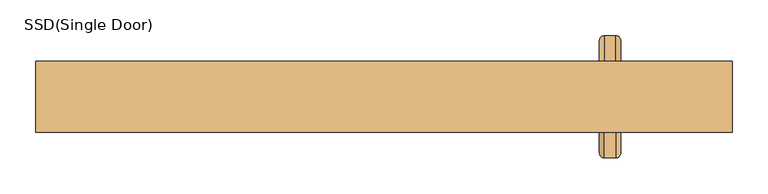
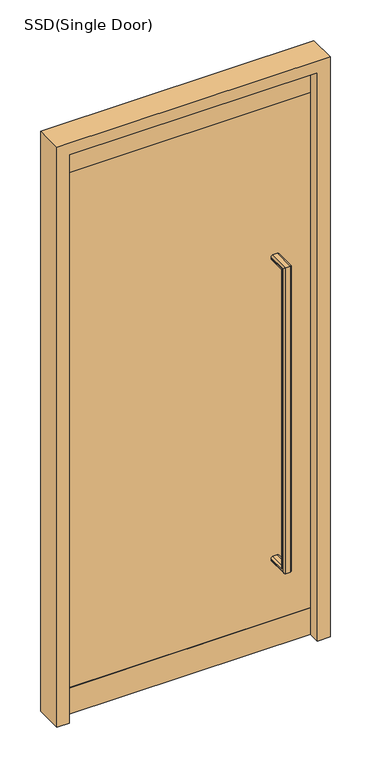
"""IFC4 building model written with IfcOpenShell, lengths in millimetres: door geometry, SSD(Single Door) : H_DR_AR B12_Door_Single_Glass_W1000xH2200_SSD-1."""

from ifc_helpers import new_model, si_unit, frame, origin, origin_with_axes, place, context, project, spatial, polyline, circle_curve, ellipse_curve, outline, extrude, source, transform, mapped, element, save
from ifc_brep_helpers import plane_surface, cylinder_surface, advanced_brep


def ssd_single_door_4e4cf73e(model_context):
    return source(origin(), model_context, "Body", "SolidModel", [
        extrude(outline(polyline([(0.0, -490.0), (0.0, -445.0), (2155.0, -445.0), (2155.0, 445.0), (0.0, 445.0), (0.0, 490.0), (2200.0, 490.0), (2200.0, -490.0), (0.0, -490.0)])), frame((0.0, -50.0, 0.0), z_axis=(0.0, 1.0, 0.0), x_axis=(0.0, 0.0, 1.0)), (0.0, 0.0, 1.0), 100.0),
        advanced_brep(
        [(310.0, -6.0, 1485.0), (326.0, -6.0, 1485.0), (333.0, -6.0, 1478.0), (333.0, -6.0, 1475.0), (326.0, -6.0, 1468.0), (310.0, -6.0, 1468.0), (303.0, -6.0, 1475.0), (303.0, -6.0, 1478.0), (310.0, -6.0, 325.0), (303.0, -6.0, 332.0), (303.0, -6.0, 335.0), (310.0, -6.0, 342.0), (326.0, -6.0, 342.0), (333.0, -6.0, 335.0), (333.0, -6.0, 332.0), (326.0, -6.0, 325.0), (310.0, -86.0, 1485.0), (326.0, -86.0, 1485.0), (333.0, -79.0, 1478.0), (333.0, -79.0, 332.0), (333.0, -76.0, 335.0), (333.0, -76.0, 1475.0), (326.0, -69.0, 1468.0), (310.0, -69.0, 1468.0), (303.0, -76.0, 1475.0), (303.0, -76.0, 335.0), (303.0, -79.0, 332.0), (303.0, -79.0, 1478.0), (310.0, -86.0, 325.0), (326.0, -86.0, 325.0), (326.0, -69.0, 342.0), (310.0, -69.0, 342.0)],
        [
            (0, 1),
            (1, 2, circle_curve(frame((326.0, -6.0, 1478.0), z_axis=(0.0, 1.0, 0.0), x_axis=(0.0, 0.0, -1.0)), 7.0)),
            (2, 3),
            (3, 4, circle_curve(frame((326.0, -6.0, 1475.0), z_axis=(0.0, 1.0, 0.0), x_axis=(0.0, 0.0, -1.0)), 7.0)),
            (4, 5),
            (5, 6, circle_curve(frame((310.0, -6.0, 1475.0), z_axis=(0.0, 1.0, 0.0), x_axis=(0.0, 0.0, -1.0)), 7.0)),
            (6, 7),
            (7, 0, circle_curve(frame((310.0, -6.0, 1478.0), z_axis=(0.0, 1.0, 0.0), x_axis=(0.0, 0.0, -1.0)), 7.0)),
            (8, 9, circle_curve(frame((310.0, -6.0, 332.0), z_axis=(0.0, 1.0, 0.0), x_axis=(0.0, 0.0, 1.0)), 7.0)),
            (9, 10),
            (10, 11, circle_curve(frame((310.0, -6.0, 335.0), z_axis=(0.0, 1.0, 0.0), x_axis=(0.0, 0.0, 1.0)), 7.0)),
            (11, 12),
            (12, 13, circle_curve(frame((326.0, -6.0, 335.0), z_axis=(0.0, 1.0, 0.0), x_axis=(0.0, 0.0, 1.0)), 7.0)),
            (13, 14),
            (14, 15, circle_curve(frame((326.0, -6.0, 332.0), z_axis=(0.0, 1.0, 0.0), x_axis=(0.0, 0.0, 1.0)), 7.0)),
            (15, 8),
            (0, 16),
            (16, 17),
            (17, 1),
            (17, 18, ellipse_curve(frame((326.0, -79.0, 1478.0), z_axis=(0.0, 0.7071067811865475, 0.7071067811865475), x_axis=(0.0, 0.7071067811865476, -0.7071067811865474)), 9.8994949, 7.0)),
            (18, 2),
            (18, 19),
            (19, 14),
            (13, 20),
            (20, 21),
            (21, 3),
            (21, 22, ellipse_curve(frame((326.0, -76.0, 1475.0), z_axis=(0.0, 0.7071067811865475, 0.7071067811865475), x_axis=(0.0, 0.7071067811865476, -0.7071067811865474)), 9.8994949, 7.0)),
            (22, 4),
            (22, 23),
            (23, 5),
            (23, 24, ellipse_curve(frame((310.0, -76.0, 1475.0), z_axis=(0.0, 0.7071067811865475, 0.7071067811865475), x_axis=(0.0, 0.7071067811865476, -0.7071067811865474)), 9.8994949, 7.0)),
            (24, 6),
            (24, 25),
            (25, 10),
            (9, 26),
            (26, 27),
            (27, 7),
            (27, 16, ellipse_curve(frame((310.0, -79.0, 1478.0), z_axis=(0.0, 0.7071067811865475, 0.7071067811865475), x_axis=(0.0, 0.7071067811865476, -0.7071067811865474)), 9.8994949, 7.0)),
            (16, 28),
            (28, 29),
            (29, 17),
            (29, 19, ellipse_curve(frame((326.0, -79.0, 332.0), z_axis=(0.0, -0.7071067811865475, 0.7071067811865475), x_axis=(0.0, 0.7071067811865474, 0.7071067811865476)), 9.8994949, 7.0)),
            (20, 30, ellipse_curve(frame((326.0, -76.0, 335.0), z_axis=(0.0, -0.7071067811865475, 0.7071067811865475), x_axis=(0.0, 0.7071067811865474, 0.7071067811865476)), 9.8994949, 7.0)),
            (30, 22),
            (30, 31),
            (31, 23),
            (31, 25, ellipse_curve(frame((310.0, -76.0, 335.0), z_axis=(0.0, -0.7071067811865475, 0.7071067811865475), x_axis=(0.0, 0.7071067811865474, 0.7071067811865476)), 9.8994949, 7.0)),
            (26, 28, ellipse_curve(frame((310.0, -79.0, 332.0), z_axis=(0.0, -0.7071067811865475, 0.7071067811865475), x_axis=(0.0, 0.7071067811865474, 0.7071067811865476)), 9.8994949, 7.0)),
            (28, 8),
            (15, 29),
            (12, 30),
            (11, 31),
        ],
        [
            plane_surface(frame((0.0, -6.0, 1485.0), z_axis=(0.0, 1.0, 0.0), x_axis=(1.0, 0.0, 0.0))),
            plane_surface(frame((0.0, -6.0, 325.0), z_axis=(0.0, 1.0, 0.0), x_axis=(1.0, 0.0, 0.0))),
            plane_surface(frame((310.0, -6.0, 1485.0), z_axis=(0.0, 0.0, 1.0), x_axis=(0.0, -1.0, 0.0))),
            cylinder_surface(frame((326.0, -6.0, 1478.0), z_axis=(0.0, 1.0, 0.0), x_axis=(0.0, 0.0, -1.0)), 7.0),
            plane_surface(frame((333.0, -6.0, 1478.0), z_axis=(1.0, 0.0, 0.0), x_axis=(0.0, -1.0, 0.0))),
            cylinder_surface(frame((326.0, -6.0, 1475.0), z_axis=(0.0, 1.0, 0.0), x_axis=(0.0, 0.0, -1.0)), 7.0),
            plane_surface(frame((326.0, -6.0, 1468.0), z_axis=(0.0, 0.0, -1.0), x_axis=(0.0, -1.0, 0.0))),
            cylinder_surface(frame((310.0, -6.0, 1475.0), z_axis=(0.0, 1.0, 0.0), x_axis=(0.0, 0.0, -1.0)), 7.0),
            plane_surface(frame((303.0, -6.0, 1475.0), z_axis=(-1.0, 0.0, 0.0), x_axis=(0.0, -1.0, 0.0))),
            cylinder_surface(frame((310.0, -6.0, 1478.0), z_axis=(0.0, 1.0, 0.0), x_axis=(0.0, 0.0, -1.0)), 7.0),
            plane_surface(frame((310.0, -86.0, 1485.0), z_axis=(0.0, -1.0, 0.0), x_axis=(0.0, 0.0, -1.0))),
            cylinder_surface(frame((326.0, -79.0, 1485.0), z_axis=(0.0, 0.0, 1.0), x_axis=(0.0, 1.0, 0.0)), 7.0),
            cylinder_surface(frame((326.0, -76.0, 1485.0), z_axis=(0.0, 0.0, 1.0), x_axis=(0.0, 1.0, 0.0)), 7.0),
            plane_surface(frame((326.0, -69.0, 1468.0), z_axis=(0.0, 1.0, 0.0), x_axis=(0.0, 0.0, -1.0))),
            cylinder_surface(frame((310.0, -76.0, 1485.0), z_axis=(0.0, 0.0, 1.0), x_axis=(0.0, 1.0, 0.0)), 7.0),
            cylinder_surface(frame((310.0, -79.0, 1485.0), z_axis=(0.0, 0.0, 1.0), x_axis=(0.0, 1.0, 0.0)), 7.0),
            plane_surface(frame((310.0, -86.0, 325.0), z_axis=(0.0, 0.0, -1.0), x_axis=(0.0, 1.0, 0.0))),
            cylinder_surface(frame((326.0, -86.0, 332.0), z_axis=(0.0, -1.0, 0.0), x_axis=(0.0, 0.0, 1.0)), 7.0),
            cylinder_surface(frame((326.0, -86.0, 335.0), z_axis=(0.0, -1.0, 0.0), x_axis=(0.0, 0.0, 1.0)), 7.0),
            plane_surface(frame((326.0, -69.0, 342.0), z_axis=(0.0, 0.0, 1.0), x_axis=(0.0, 1.0, 0.0))),
            cylinder_surface(frame((310.0, -86.0, 335.0), z_axis=(0.0, -1.0, 0.0), x_axis=(0.0, 0.0, 1.0)), 7.0),
            cylinder_surface(frame((310.0, -86.0, 332.0), z_axis=(0.0, -1.0, 0.0), x_axis=(0.0, 0.0, 1.0)), 7.0),
        ],
        [
            (0, [[1, 2, 3, 4, 5, 6, 7, 8]]),
            (1, [[9, 10, 11, 12, 13, 14, 15, 16]]),
            (2, [[-1, 17, 18, 19]]),
            (3, [[-2, -19, 20, 21]]),
            (4, [[-3, -21, 22, 23, -14, 24, 25, 26]]),
            (5, [[-4, -26, 27, 28]]),
            (6, [[-5, -28, 29, 30]]),
            (7, [[-6, -30, 31, 32]]),
            (8, [[-7, -32, 33, 34, -10, 35, 36, 37]]),
            (9, [[-8, -37, 38, -17]]),
            (10, [[-18, 39, 40, 41]]),
            (11, [[-20, -41, 42, -22]]),
            (12, [[-27, -25, 43, 44]]),
            (13, [[-29, -44, 45, 46]]),
            (14, [[-31, -46, 47, -33]]),
            (15, [[-38, -36, 48, -39]]),
            (16, [[-40, 49, -16, 50]]),
            (17, [[-42, -50, -15, -23]]),
            (18, [[-43, -24, -13, 51]]),
            (19, [[-45, -51, -12, 52]]),
            (20, [[-47, -52, -11, -34]]),
            (21, [[-48, -35, -9, -49]]),
        ],
    ),
        advanced_brep(
        [(310.0, 6.0, 1485.0), (303.0, 6.0, 1478.0), (303.0, 6.0, 1475.0), (310.0, 6.0, 1468.0), (326.0, 6.0, 1468.0), (333.0, 6.0, 1475.0), (333.0, 6.0, 1478.0), (326.0, 6.0, 1485.0), (310.0, 6.0, 325.0), (326.0, 6.0, 325.0), (333.0, 6.0, 332.0), (333.0, 6.0, 335.0), (326.0, 6.0, 342.0), (310.0, 6.0, 342.0), (303.0, 6.0, 335.0), (303.0, 6.0, 332.0), (310.0, 86.0, 1485.0), (303.0, 79.0, 1478.0), (303.0, 79.0, 332.0), (303.0, 76.0, 335.0), (303.0, 76.0, 1475.0), (310.0, 69.0, 1468.0), (326.0, 69.0, 1468.0), (333.0, 76.0, 1475.0), (333.0, 76.0, 335.0), (333.0, 79.0, 332.0), (333.0, 79.0, 1478.0), (326.0, 86.0, 1485.0), (310.0, 86.0, 325.0), (310.0, 69.0, 342.0), (326.0, 69.0, 342.0), (326.0, 86.0, 325.0)],
        [
            (0, 1, circle_curve(frame((310.0, 6.0, 1478.0), z_axis=(0.0, -1.0, 0.0), x_axis=(0.0, 0.0, 1.0)), 7.0)),
            (1, 2),
            (2, 3, circle_curve(frame((310.0, 6.0, 1475.0), z_axis=(0.0, -1.0, 0.0), x_axis=(0.0, 0.0, 1.0)), 7.0)),
            (3, 4),
            (4, 5, circle_curve(frame((326.0, 6.0, 1475.0), z_axis=(0.0, -1.0, 0.0), x_axis=(0.0, 0.0, 1.0)), 7.0)),
            (5, 6),
            (6, 7, circle_curve(frame((326.0, 6.0, 1478.0), z_axis=(0.0, -1.0, 0.0), x_axis=(0.0, 0.0, 1.0)), 7.0)),
            (7, 0),
            (8, 9),
            (9, 10, circle_curve(frame((326.0, 6.0, 332.0), z_axis=(0.0, -1.0, 0.0), x_axis=(0.0, 0.0, -1.0)), 7.0)),
            (10, 11),
            (11, 12, circle_curve(frame((326.0, 6.0, 335.0), z_axis=(0.0, -1.0, 0.0), x_axis=(0.0, 0.0, -1.0)), 7.0)),
            (12, 13),
            (13, 14, circle_curve(frame((310.0, 6.0, 335.0), z_axis=(0.0, -1.0, 0.0), x_axis=(0.0, 0.0, -1.0)), 7.0)),
            (14, 15),
            (15, 8, circle_curve(frame((310.0, 6.0, 332.0), z_axis=(0.0, -1.0, 0.0), x_axis=(0.0, 0.0, -1.0)), 7.0)),
            (0, 16),
            (16, 17, ellipse_curve(frame((310.0, 79.0, 1478.0), z_axis=(0.0, -0.7071067811865475, 0.7071067811865475), x_axis=(0.0, -0.7071067811865476, -0.7071067811865474)), 9.8994949, 7.0)),
            (17, 1),
            (17, 18),
            (18, 15),
            (14, 19),
            (19, 20),
            (20, 2),
            (20, 21, ellipse_curve(frame((310.0, 76.0, 1475.0), z_axis=(0.0, -0.7071067811865475, 0.7071067811865475), x_axis=(0.0, -0.7071067811865476, -0.7071067811865474)), 9.8994949, 7.0)),
            (21, 3),
            (21, 22),
            (22, 4),
            (22, 23, ellipse_curve(frame((326.0, 76.0, 1475.0), z_axis=(0.0, -0.7071067811865475, 0.7071067811865475), x_axis=(0.0, -0.7071067811865476, -0.7071067811865474)), 9.8994949, 7.0)),
            (23, 5),
            (23, 24),
            (24, 11),
            (10, 25),
            (25, 26),
            (26, 6),
            (26, 27, ellipse_curve(frame((326.0, 79.0, 1478.0), z_axis=(0.0, -0.7071067811865475, 0.7071067811865475), x_axis=(0.0, -0.7071067811865476, -0.7071067811865474)), 9.8994949, 7.0)),
            (27, 7),
            (27, 16),
            (16, 28),
            (28, 18, ellipse_curve(frame((310.0, 79.0, 332.0), z_axis=(0.0, 0.7071067811865475, 0.7071067811865475), x_axis=(0.0, -0.7071067811865474, 0.7071067811865476)), 9.8994949, 7.0)),
            (19, 29, ellipse_curve(frame((310.0, 76.0, 335.0), z_axis=(0.0, 0.7071067811865475, 0.7071067811865475), x_axis=(0.0, -0.7071067811865474, 0.7071067811865476)), 9.8994949, 7.0)),
            (29, 21),
            (29, 30),
            (30, 22),
            (30, 24, ellipse_curve(frame((326.0, 76.0, 335.0), z_axis=(0.0, 0.7071067811865475, 0.7071067811865475), x_axis=(0.0, -0.7071067811865474, 0.7071067811865476)), 9.8994949, 7.0)),
            (25, 31, ellipse_curve(frame((326.0, 79.0, 332.0), z_axis=(0.0, 0.7071067811865475, 0.7071067811865475), x_axis=(0.0, -0.7071067811865474, 0.7071067811865476)), 9.8994949, 7.0)),
            (31, 27),
            (31, 28),
            (28, 8),
            (13, 29),
            (12, 30),
            (9, 31),
        ],
        [
            plane_surface(frame((0.0, 6.0, 1485.0), z_axis=(0.0, -1.0, 0.0), x_axis=(1.0, 0.0, 0.0))),
            plane_surface(frame((0.0, 6.0, 325.0), z_axis=(0.0, -1.0, 0.0), x_axis=(1.0, 0.0, 0.0))),
            cylinder_surface(frame((310.0, 6.0, 1478.0), z_axis=(0.0, -1.0, 0.0), x_axis=(0.0, 0.0, 1.0)), 7.0),
            plane_surface(frame((303.0, 6.0, 1478.0), z_axis=(-1.0, 0.0, 0.0), x_axis=(0.0, 1.0, 0.0))),
            cylinder_surface(frame((310.0, 6.0, 1475.0), z_axis=(0.0, -1.0, 0.0), x_axis=(0.0, 0.0, 1.0)), 7.0),
            plane_surface(frame((310.0, 6.0, 1468.0), z_axis=(0.0, 0.0, -1.0), x_axis=(0.0, 1.0, 0.0))),
            cylinder_surface(frame((326.0, 6.0, 1475.0), z_axis=(0.0, -1.0, 0.0), x_axis=(0.0, 0.0, 1.0)), 7.0),
            plane_surface(frame((333.0, 6.0, 1475.0), z_axis=(1.0, 0.0, 0.0), x_axis=(0.0, 1.0, 0.0))),
            cylinder_surface(frame((326.0, 6.0, 1478.0), z_axis=(0.0, -1.0, 0.0), x_axis=(0.0, 0.0, 1.0)), 7.0),
            plane_surface(frame((326.0, 6.0, 1485.0), z_axis=(0.0, 0.0, 1.0), x_axis=(0.0, 1.0, 0.0))),
            cylinder_surface(frame((310.0, 79.0, 1485.0), z_axis=(0.0, 0.0, 1.0), x_axis=(0.0, 1.0, 0.0)), 7.0),
            cylinder_surface(frame((310.0, 76.0, 1485.0), z_axis=(0.0, 0.0, 1.0), x_axis=(0.0, 1.0, 0.0)), 7.0),
            plane_surface(frame((310.0, 69.0, 1468.0), z_axis=(0.0, -1.0, 0.0), x_axis=(0.0, 0.0, -1.0))),
            cylinder_surface(frame((326.0, 76.0, 1485.0), z_axis=(0.0, 0.0, 1.0), x_axis=(0.0, 1.0, 0.0)), 7.0),
            cylinder_surface(frame((326.0, 79.0, 1485.0), z_axis=(0.0, 0.0, 1.0), x_axis=(0.0, 1.0, 0.0)), 7.0),
            plane_surface(frame((326.0, 86.0, 1485.0), z_axis=(0.0, 1.0, 0.0), x_axis=(0.0, 0.0, -1.0))),
            cylinder_surface(frame((310.0, 86.0, 332.0), z_axis=(0.0, 1.0, 0.0), x_axis=(0.0, 0.0, -1.0)), 7.0),
            cylinder_surface(frame((310.0, 86.0, 335.0), z_axis=(0.0, 1.0, 0.0), x_axis=(0.0, 0.0, -1.0)), 7.0),
            plane_surface(frame((310.0, 69.0, 342.0), z_axis=(0.0, 0.0, 1.0), x_axis=(0.0, -1.0, 0.0))),
            cylinder_surface(frame((326.0, 86.0, 335.0), z_axis=(0.0, 1.0, 0.0), x_axis=(0.0, 0.0, -1.0)), 7.0),
            cylinder_surface(frame((326.0, 86.0, 332.0), z_axis=(0.0, 1.0, 0.0), x_axis=(0.0, 0.0, -1.0)), 7.0),
            plane_surface(frame((326.0, 86.0, 325.0), z_axis=(0.0, 0.0, -1.0), x_axis=(0.0, -1.0, 0.0))),
        ],
        [
            (0, [[1, 2, 3, 4, 5, 6, 7, 8]]),
            (1, [[9, 10, 11, 12, 13, 14, 15, 16]]),
            (2, [[-1, 17, 18, 19]]),
            (3, [[-2, -19, 20, 21, -15, 22, 23, 24]]),
            (4, [[-3, -24, 25, 26]]),
            (5, [[-4, -26, 27, 28]]),
            (6, [[-5, -28, 29, 30]]),
            (7, [[-6, -30, 31, 32, -11, 33, 34, 35]]),
            (8, [[-7, -35, 36, 37]]),
            (9, [[-8, -37, 38, -17]]),
            (10, [[-18, 39, 40, -20]]),
            (11, [[-25, -23, 41, 42]]),
            (12, [[-27, -42, 43, 44]]),
            (13, [[-29, -44, 45, -31]]),
            (14, [[-36, -34, 46, 47]]),
            (15, [[-38, -47, 48, -39]]),
            (16, [[-40, 49, -16, -21]]),
            (17, [[-41, -22, -14, 50]]),
            (18, [[-43, -50, -13, 51]]),
            (19, [[-45, -51, -12, -32]]),
            (20, [[-46, -33, -10, 52]]),
            (21, [[-48, -52, -9, -49]]),
        ],
    ),
        extrude(outline(polyline([(445.0, -6.0), (-445.0, -6.0), (-445.0, 6.0), (445.0, 6.0), (445.0, -6.0)])), frame((0.0, 0.0, 100.0), z_axis=(0.0, 0.0, 1.0), x_axis=(1.0, 0.0, 0.0)), (0.0, 0.0, 1.0), 1955.0),
        extrude(outline(polyline([(445.0, -8.0), (-445.0, -8.0), (-445.0, 8.0), (445.0, 8.0), (445.0, -8.0)])), frame((0.0, 0.0, 2055.0), z_axis=(0.0, 0.0, 1.0), x_axis=(1.0, 0.0, 0.0)), (0.0, 0.0, 1.0), 100.0),
        extrude(outline(polyline([(445.0, -8.0), (-445.0, -8.0), (-445.0, 8.0), (445.0, 8.0), (445.0, -8.0)])), origin_with_axes(), (0.0, 0.0, 1.0), 100.0),
    ])


if __name__ == "__main__":
    model = new_model("IFC4")
    model_context = context("Model", 3, world=origin())
    ifc_project = project(units=[si_unit("LENGTHUNIT", "METRE", prefix="MILLI")], contexts=[model_context])
    site = spatial("IfcSite", under=ifc_project)
    building = spatial("IfcBuilding", under=site)
    placement = place(None, origin())
    ssd_single_door_shape = ssd_single_door_4e4cf73e(model_context)
    element("IfcDoor", 1, ObjectType="SSD(Single Door) : H_DR_AR B12_Door_Single_Glass_W1000xH2200_SSD-1", at=placement, inside=building, context=model_context, shape_type="MappedRepresentation", body=[
        mapped(ssd_single_door_shape, transform((0.0, 0.0, 0.0), x_axis=(1.0, 0.0, 0.0), y_axis=(0.0, 1.0, 0.0), z_axis=(0.0, 0.0, 1.0))),
    ])
    save(model, "model.ifc")

# Revit data of these elements
# Type "SSD(Single Door) : H_DR_AR B12_Door_Single_Glass_W1000xH2200_SSD-1"
#   Type Mark = "452"
#   Type Comments = "SSD"
#   Analytic Construction = "<None>"
#   Thickness = 45 mm
#   Plan Door Swing2 = 890 mm
#   Plan Door Swing = 1780 mm
#   Glass Thk = 12 mm
#   Frame THK = 100 mm
#   Frame Projection Ext. = 25 mm
#   Frame Projection Int. = 25 mm
#   Frame Width = 75 mm
#   Height = 2200 mm
#   Width = 980 mm
#   Center Door [instance default] = 100 mm
#   Define Thermal Properties by = 1
#   Function = (empty or 0)
#   Wall Closure = (empty or 0)
# Element 1 (IfcDoor, "SSD(Single Door) : H_DR_AR B12_Door_Single_Glass_W1000xH2200_SSD-1")
#   Center Door = 0 mm
#   Materials on its faces: "Stainless Steel", "Glass"
# Materials
#   "Stainless Steel": class "Metal", colour RGB 189 187 185, transparency 0, Description = "Stainless Steel 18/8", Cost = 0
#   "Glass": class "Glass", colour RGB 218 227 224, transparency 0.85, Description = "Soda Lime Glass", Cost = 0
